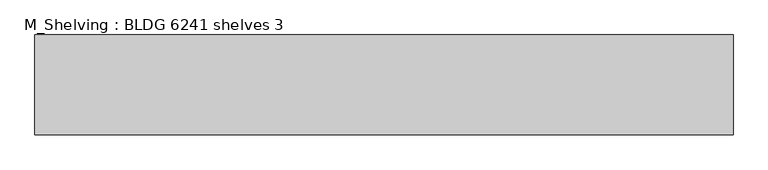
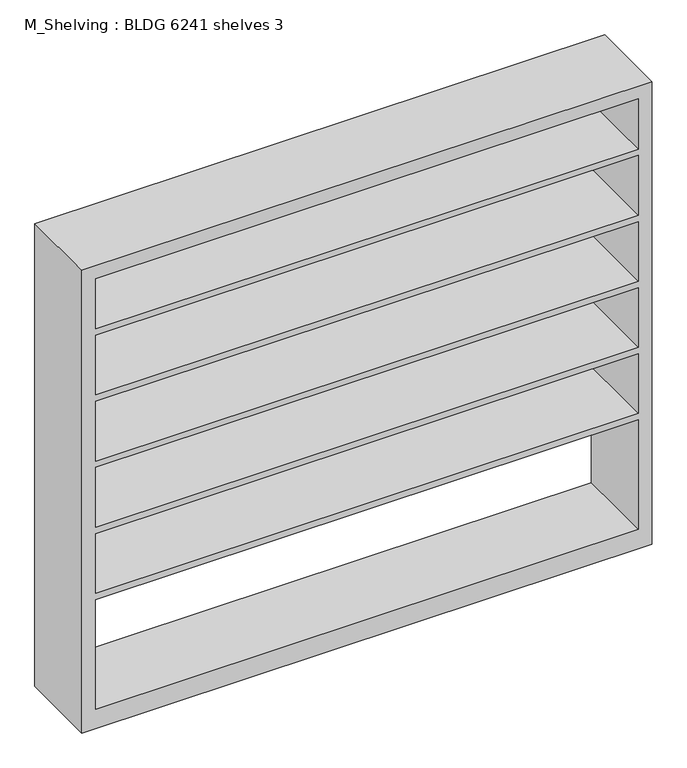
"""IFC4 building model written with IfcOpenShell, lengths in millimetres: furniture geometry, M_Shelving : BLDG 6241 shelves 3."""

from ifc_helpers import new_model, si_unit, frame, origin, place, context, project, spatial, polyline, outline, extrude, source, transform, mapped, element, save


def m_shelving_bldg_6241_shelves_3_923b8557(model_context):
    return source(origin(), model_context, "Body", "SweptSolid", [
        extrude(outline(polyline([(0.0, 1066.8992188), (1830.0, 1066.8992188), (1830.0, -1066.8992188), (0.0, -1066.8992188), (0.0, 1066.8992188)]), holes=[polyline([(1779.2, 1016.0992188), (1581.2714286, 1016.0992188), (1581.2714286, -1016.0992188), (1779.2, -1016.0992188), (1779.2, 1016.0992188)]), polyline([(76.2, 1016.0992188), (76.2, -1016.0992188), (510.1571429, -1016.0992188), (510.1571429, 1016.0992188), (76.2, 1016.0992188)]), polyline([(1058.4142857, -1016.0992188), (1294.4428571, -1016.0992188), (1294.4428571, 1016.0992188), (1058.4142857, 1016.0992188), (1058.4142857, -1016.0992188)]), polyline([(1555.8714286, 1016.0992188), (1319.8428571, 1016.0992188), (1319.8428571, -1016.0992188), (1555.8714286, -1016.0992188), (1555.8714286, 1016.0992188)]), polyline([(1033.0142857, 1016.0992188), (796.9857143, 1016.0992188), (796.9857143, -1016.0992188), (1033.0142857, -1016.0992188), (1033.0142857, 1016.0992188)]), polyline([(771.5857143, 1016.0992188), (535.5571429, 1016.0992188), (535.5571429, -1016.0992188), (771.5857143, -1016.0992188), (771.5857143, 1016.0992188)])]), frame((0.0, -457.2, 0.0), z_axis=(0.0, 1.0, 0.0), x_axis=(0.0, 0.0, 1.0)), (0.0, 0.0, 1.0), 304.8),
    ])


if __name__ == "__main__":
    model = new_model("IFC4")
    model_context = context("Model", 3, world=origin())
    ifc_project = project(units=[si_unit("LENGTHUNIT", "METRE", prefix="MILLI")], contexts=[model_context])
    site = spatial("IfcSite", under=ifc_project)
    building = spatial("IfcBuilding", under=site)
    placement = place(None, origin())
    m_shelving_bldg_6241_shelves_3_shape = m_shelving_bldg_6241_shelves_3_923b8557(model_context)
    element("IfcFurniture", 1, ObjectType="M_Shelving : BLDG 6241 shelves 3", at=placement, inside=building, context=model_context, shape_type="MappedRepresentation", body=[
        mapped(m_shelving_bldg_6241_shelves_3_shape, transform((0.0, 0.0, 0.0), x_axis=(1.0, 0.0, 0.0), y_axis=(0.0, 1.0, 0.0), z_axis=(0.0, 0.0, 1.0))),
    ])
    save(model, "model.ifc")

# Revit data of these elements
# Type "M_Shelving : BLDG 6241 shelves 3"
#   Depth = 1' - 0"
#   Height = 6' - 0.04724"
#   Width = 7' - 0 1/128"
#   Material = Birch
#   Default Elevation = 0
# Element 1 (IfcFurniture, "M_Shelving : BLDG 6241 shelves 3")
#   Materials on its faces: "Birch"
# Materials
#   "Birch": class "Wood", colour RGB 224 178 126, transparency 0, Description = "Betula Alleghaniensis", Cost = 0
